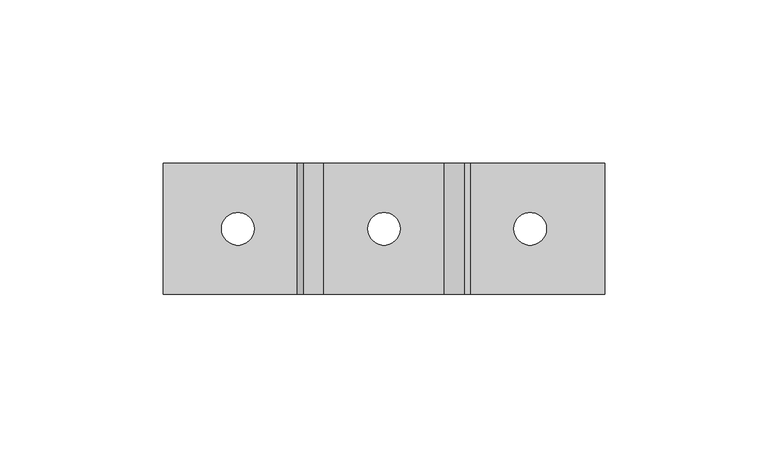
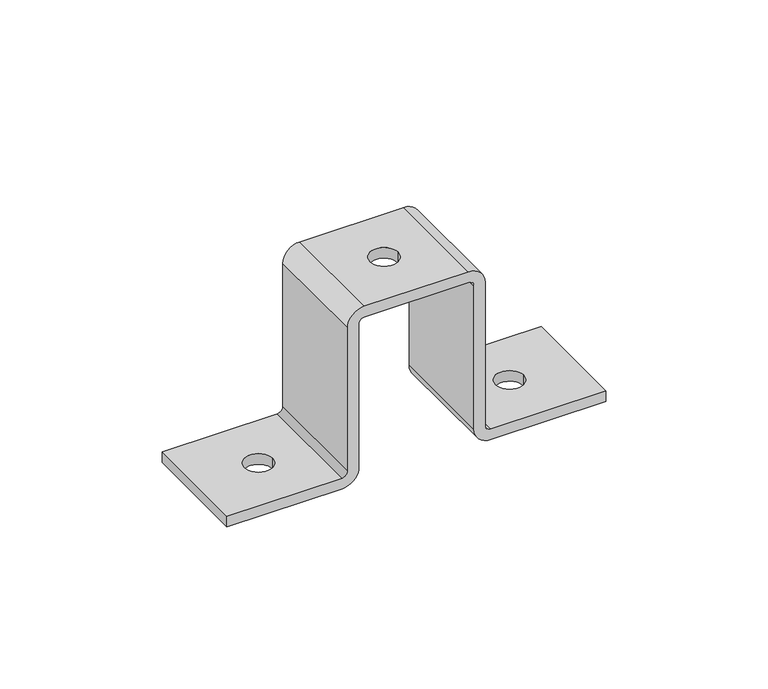
"""IFC4 building model written with IfcOpenShell, lengths in millimetres: proxy geometry, ▶ TN_Скоба соединительная (сборка тип 1) : ▶ TN_Скоба соединительная (сборка тип 1)."""

from ifc_helpers import new_model, si_unit, frame, origin, place, context, project, spatial, polyline, circle_curve, source, transform, mapped, element, save
from ifc_brep_helpers import plane_surface, cylinder_surface, revolved_surface, advanced_brep


def generic_models_d1ea9576(model_context):
    return source(origin(), model_context, "Body", "AdvancedBrep", [
        advanced_brep(
        [(-26.5, -20.0, 0.0), (-20.5, -20.0, 6.0), (-20.5, -20.0, 60.0), (-18.5, -20.0, 62.0), (18.5, -20.0, 62.0), (20.5, -20.0, 60.0), (20.5, -20.0, 6.0), (26.5, -20.0, 0.0), (67.5, -20.0, 0.0), (67.5, -20.0, 4.0), (26.5, -20.0, 4.0), (24.5, -20.0, 6.0), (24.5, -20.0, 60.0), (18.5, -20.0, 66.0), (-18.5, -20.0, 66.0), (-24.5, -20.0, 60.0), (-24.5, -20.0, 6.0), (-26.5, -20.0, 4.0), (-67.5, -20.0, 4.0), (-67.5, -20.0, 0.0), (-26.5, 20.0, 0.0), (-67.5, 20.0, 0.0), (-67.5, 20.0, 4.0), (-26.5, 20.0, 4.0), (-24.5, 20.0, 6.0), (-24.5, 20.0, 60.0), (-18.5, 20.0, 66.0), (18.5, 20.0, 66.0), (24.5, 20.0, 60.0), (24.5, 20.0, 6.0), (26.5, 20.0, 4.0), (67.5, 20.0, 4.0), (67.5, 20.0, 0.0), (26.5, 20.0, 0.0), (20.5, 20.0, 6.0), (20.5, 20.0, 60.0), (18.5, 20.0, 62.0), (-18.5, 20.0, 62.0), (-20.5, 20.0, 60.0), (-20.5, 20.0, 6.0), (-5.0, 0.0, 62.0), (5.0, 0.0, 62.0), (39.7162685, 0.0, 0.0), (49.7162685, 0.0, 0.0), (49.7162685, 0.0, 4.0), (39.7162685, 0.0, 4.0), (5.0, 0.0, 66.0), (-5.0, 0.0, 66.0), (-39.7162685, 0.0, 4.0), (-49.7162685, 0.0, 4.0), (-49.7162685, 0.0, 0.0), (-39.7162685, 0.0, 0.0)],
        [
            (0, 1, circle_curve(frame((-26.5, -20.0, 6.0), z_axis=(0.0, -1.0, 0.0), x_axis=(0.0, 0.0, -1.0)), 6.0)),
            (1, 2),
            (2, 3, circle_curve(frame((-18.5, -20.0, 60.0), z_axis=(0.0, 1.0, 0.0), x_axis=(0.0, 0.0, -1.0)), 2.0)),
            (3, 4),
            (4, 5, circle_curve(frame((18.5, -20.0, 60.0), z_axis=(0.0, 1.0, 0.0), x_axis=(0.0, 0.0, -1.0)), 2.0)),
            (5, 6),
            (6, 7, circle_curve(frame((26.5, -20.0, 6.0), z_axis=(0.0, -1.0, 0.0), x_axis=(0.0, 0.0, -1.0)), 6.0)),
            (7, 8),
            (8, 9),
            (9, 10),
            (10, 11, circle_curve(frame((26.5, -20.0, 6.0), z_axis=(0.0, 1.0, 0.0), x_axis=(0.0, 0.0, -1.0)), 2.0)),
            (11, 12),
            (12, 13, circle_curve(frame((18.5, -20.0, 60.0), z_axis=(0.0, -1.0, 0.0), x_axis=(0.0, 0.0, -1.0)), 6.0)),
            (13, 14),
            (14, 15, circle_curve(frame((-18.5, -20.0, 60.0), z_axis=(0.0, -1.0, 0.0), x_axis=(0.0, 0.0, -1.0)), 6.0)),
            (15, 16),
            (16, 17, circle_curve(frame((-26.5, -20.0, 6.0), z_axis=(0.0, 1.0, 0.0), x_axis=(0.0, 0.0, -1.0)), 2.0)),
            (17, 18),
            (18, 19),
            (19, 0),
            (20, 21),
            (21, 22),
            (22, 23),
            (23, 24, circle_curve(frame((-26.5, 20.0, 6.0), z_axis=(0.0, -1.0, 0.0), x_axis=(0.0, 0.0, -1.0)), 2.0)),
            (24, 25),
            (25, 26, circle_curve(frame((-18.5, 20.0, 60.0), z_axis=(0.0, 1.0, 0.0), x_axis=(0.0, 0.0, -1.0)), 6.0)),
            (26, 27),
            (27, 28, circle_curve(frame((18.5, 20.0, 60.0), z_axis=(0.0, 1.0, 0.0), x_axis=(0.0, 0.0, -1.0)), 6.0)),
            (28, 29),
            (29, 30, circle_curve(frame((26.5, 20.0, 6.0), z_axis=(0.0, -1.0, 0.0), x_axis=(0.0, 0.0, -1.0)), 2.0)),
            (30, 31),
            (31, 32),
            (32, 33),
            (33, 34, circle_curve(frame((26.5, 20.0, 6.0), z_axis=(0.0, 1.0, 0.0), x_axis=(0.0, 0.0, -1.0)), 6.0)),
            (34, 35),
            (35, 36, circle_curve(frame((18.5, 20.0, 60.0), z_axis=(0.0, -1.0, 0.0), x_axis=(0.0, 0.0, -1.0)), 2.0)),
            (36, 37),
            (37, 38, circle_curve(frame((-18.5, 20.0, 60.0), z_axis=(0.0, -1.0, 0.0), x_axis=(0.0, 0.0, -1.0)), 2.0)),
            (38, 39),
            (39, 20, circle_curve(frame((-26.5, 20.0, 6.0), z_axis=(0.0, 1.0, 0.0), x_axis=(0.0, 0.0, -1.0)), 6.0)),
            (0, 20),
            (39, 1),
            (38, 2),
            (37, 3),
            (36, 4),
            (40, 41, circle_curve(frame((0.0, 0.0, 62.0), z_axis=(0.0, 0.0, 1.0), x_axis=(1.0, 0.0, 0.0)), 5.0)),
            (41, 40, circle_curve(frame((0.0, 0.0, 62.0), z_axis=(0.0, 0.0, 1.0), x_axis=(1.0, 0.0, 0.0)), 5.0)),
            (35, 5),
            (34, 6),
            (33, 7),
            (32, 8),
            (42, 43, circle_curve(frame((44.7162685, 0.0, 0.0), z_axis=(0.0, 0.0, 1.0), x_axis=(1.0, 0.0, 0.0)), 5.0)),
            (43, 42, circle_curve(frame((44.7162685, 0.0, 0.0), z_axis=(0.0, 0.0, 1.0), x_axis=(1.0, 0.0, 0.0)), 5.0)),
            (31, 9),
            (30, 10),
            (44, 45, circle_curve(frame((44.7162685, 0.0, 4.0), z_axis=(0.0, 0.0, -1.0), x_axis=(1.0, 0.0, 0.0)), 5.0)),
            (45, 44, circle_curve(frame((44.7162685, 0.0, 4.0), z_axis=(0.0, 0.0, -1.0), x_axis=(1.0, 0.0, 0.0)), 5.0)),
            (29, 11),
            (28, 12),
            (27, 13),
            (26, 14),
            (46, 47, circle_curve(frame((0.0, 0.0, 66.0), z_axis=(0.0, 0.0, -1.0), x_axis=(1.0, 0.0, 0.0)), 5.0)),
            (47, 46, circle_curve(frame((0.0, 0.0, 66.0), z_axis=(0.0, 0.0, -1.0), x_axis=(1.0, 0.0, 0.0)), 5.0)),
            (25, 15),
            (24, 16),
            (23, 17),
            (22, 18),
            (48, 49, circle_curve(frame((-44.7162685, 0.0, 4.0), z_axis=(0.0, 0.0, -1.0), x_axis=(1.0, 0.0, 0.0)), 5.0)),
            (49, 48, circle_curve(frame((-44.7162685, 0.0, 4.0), z_axis=(0.0, 0.0, -1.0), x_axis=(1.0, 0.0, 0.0)), 5.0)),
            (21, 19),
            (50, 51, circle_curve(frame((-44.7162685, 0.0, 0.0), z_axis=(0.0, 0.0, 1.0), x_axis=(1.0, 0.0, 0.0)), 5.0)),
            (51, 50, circle_curve(frame((-44.7162685, 0.0, 0.0), z_axis=(0.0, 0.0, 1.0), x_axis=(1.0, 0.0, 0.0)), 5.0)),
            (48, 51),
            (50, 49),
            (44, 43),
            (42, 45),
            (40, 47),
            (46, 41),
        ],
        [
            plane_surface(frame((0.0, -20.0, 0.0), z_axis=(0.0, -1.0, 0.0), x_axis=(0.0, 0.0, 1.0))),
            plane_surface(frame((0.0, 20.0, 0.0), z_axis=(0.0, 1.0, 0.0), x_axis=(0.0, 0.0, 1.0))),
            cylinder_surface(frame((-26.5, -20.0, 6.0), z_axis=(0.0, -1.0, 0.0), x_axis=(0.0, 0.0, -1.0)), 6.0),
            plane_surface(frame((-20.5, -20.0, 6.0), z_axis=(1.0, 0.0, 0.0), x_axis=(0.0, 1.0, 0.0))),
            revolved_surface(polyline([(-18.5, 20.0, 58.0), (-18.5, -20.0, 58.0)]), (-18.5, -20.0, 60.0), (0.0, 1.0, 0.0)),
            plane_surface(frame((-18.5, -20.0, 62.0), z_axis=(0.0, 0.0, -1.0), x_axis=(0.0, 1.0, 0.0))),
            revolved_surface(polyline([(18.5, 20.0, 58.0), (18.5, -20.0, 58.0)]), (18.5, -20.0, 60.0), (0.0, 1.0, 0.0)),
            plane_surface(frame((20.5, -20.0, 60.0), z_axis=(-1.0, 0.0, 0.0), x_axis=(0.0, 1.0, 0.0))),
            cylinder_surface(frame((26.5, -20.0, 6.0), z_axis=(0.0, -1.0, 0.0), x_axis=(0.0, 0.0, -1.0)), 6.0),
            plane_surface(frame((26.5, -20.0, 0.0), z_axis=(0.0, 0.0, -1.0), x_axis=(0.0, 1.0, 0.0))),
            plane_surface(frame((67.5, -20.0, 0.0), z_axis=(1.0, 0.0, 0.0), x_axis=(0.0, 1.0, 0.0))),
            plane_surface(frame((67.5, -20.0, 4.0), z_axis=(0.0, 0.0, 1.0), x_axis=(0.0, 1.0, 0.0))),
            revolved_surface(polyline([(26.5, 20.0, 4.0), (26.5, -20.0, 4.0)]), (26.5, -20.0, 6.0), (0.0, 1.0, 0.0)),
            plane_surface(frame((24.5, -20.0, 6.0), z_axis=(1.0, 0.0, 0.0), x_axis=(0.0, 1.0, 0.0))),
            cylinder_surface(frame((18.5, -20.0, 60.0), z_axis=(0.0, -1.0, 0.0), x_axis=(0.0, 0.0, -1.0)), 6.0),
            plane_surface(frame((18.5, -20.0, 66.0), z_axis=(0.0, 0.0, 1.0), x_axis=(0.0, 1.0, 0.0))),
            cylinder_surface(frame((-18.5, -20.0, 60.0), z_axis=(0.0, -1.0, 0.0), x_axis=(0.0, 0.0, -1.0)), 6.0),
            plane_surface(frame((-24.5, -20.0, 60.0), z_axis=(-1.0, 0.0, 0.0), x_axis=(0.0, 1.0, 0.0))),
            revolved_surface(polyline([(-26.5, 20.0, 4.0), (-26.5, -20.0, 4.0)]), (-26.5, -20.0, 6.0), (0.0, 1.0, 0.0)),
            plane_surface(frame((-26.5, -20.0, 4.0), z_axis=(0.0, 0.0, 1.0), x_axis=(0.0, 1.0, 0.0))),
            plane_surface(frame((-67.5, -20.0, 4.0), z_axis=(-1.0, 0.0, 0.0), x_axis=(0.0, 1.0, 0.0))),
            plane_surface(frame((-67.5, -20.0, 0.0), z_axis=(0.0, 0.0, -1.0), x_axis=(0.0, 1.0, 0.0))),
            revolved_surface(polyline([(-39.7162685, 0.0, 4.0), (-39.7162685, 0.0, 0.0)]), (-44.7162685, 0.0, 0.0), (0.0, 0.0, 1.0)),
            revolved_surface(polyline([(49.7162685, 0.0, 4.0), (49.7162685, 0.0, 0.0)]), (44.7162685, 0.0, 0.0), (0.0, 0.0, 1.0)),
            revolved_surface(polyline([(5.0, 0.0, 66.0), (5.0, 0.0, 62.0)]), (0.0, 0.0, 35.2036226), (0.0, 0.0, 1.0)),
        ],
        [
            (0, [[1, 2, 3, 4, 5, 6, 7, 8, 9, 10, 11, 12, 13, 14, 15, 16, 17, 18, 19, 20]]),
            (1, [[21, 22, 23, 24, 25, 26, 27, 28, 29, 30, 31, 32, 33, 34, 35, 36, 37, 38, 39, 40]]),
            (2, [[-1, 41, -40, 42]]),
            (3, [[-2, -42, -39, 43]]),
            (4, [[-3, -43, -38, 44]]),
            (5, [[-4, -44, -37, 45], [46, 47]]),
            (6, [[-5, -45, -36, 48]]),
            (7, [[-6, -48, -35, 49]]),
            (8, [[-7, -49, -34, 50]]),
            (9, [[-8, -50, -33, 51], [52, 53]]),
            (10, [[-9, -51, -32, 54]]),
            (11, [[-10, -54, -31, 55], [56, 57]]),
            (12, [[-11, -55, -30, 58]]),
            (13, [[-12, -58, -29, 59]]),
            (14, [[-13, -59, -28, 60]]),
            (15, [[-14, -60, -27, 61], [62, 63]]),
            (16, [[-15, -61, -26, 64]]),
            (17, [[-16, -64, -25, 65]]),
            (18, [[-17, -65, -24, 66]]),
            (19, [[-18, -66, -23, 67], [68, 69]]),
            (20, [[-19, -67, -22, 70]]),
            (21, [[-20, -70, -21, -41], [71, 72]]),
            (22, [[73, -71, 74, -68]]),
            (22, [[-73, -69, -74, -72]]),
            (23, [[75, -52, 76, -56]]),
            (23, [[-75, -57, -76, -53]]),
            (24, [[77, -62, 78, -46]]),
            (24, [[-77, -47, -78, -63]]),
        ],
    ),
    ])


if __name__ == "__main__":
    model = new_model("IFC4")
    model_context = context("Model", 3, world=origin())
    ifc_project = project(units=[si_unit("LENGTHUNIT", "METRE", prefix="MILLI")], contexts=[model_context])
    site = spatial("IfcSite", under=ifc_project)
    building = spatial("IfcBuilding", under=site)
    placement = place(None, origin())
    generic_models_shape = generic_models_d1ea9576(model_context)
    element("IfcBuildingElementProxy", 1, Name="▶ TN_Скоба соединительная (сборка тип 1) : ▶ TN_Скоба соединительная (сборка тип 1)", ObjectType="▶ TN_Скоба соединительная (сборка тип 1) : ▶ TN_Скоба соединительная (сборка тип 1)", at=placement, inside=building, context=model_context, shape_type="MappedRepresentation", body=[
        mapped(generic_models_shape, transform((0.0, 0.0, 0.0), x_axis=(1.0, 0.0, 0.0), y_axis=(0.0, 1.0, 0.0), z_axis=(0.0, 0.0, 1.0))),
    ])
    save(model, "model.ifc")

# Revit data of these elements
# Type "▶ TN_Скоба соединительная (сборка тип 1) : ▶ TN_Скоба соединительная (сборка тип 1)"
#   Description = "Cоединительный элемент для монтажа рам, стеллажей, каркасов для легких и средних систем. Обеспечивает устойчивое поперечное (крестовое) соединение профилей. Наиболее эффективно использования скобы, как соединителя для создания пространственных силовых, опорных каркасов и решеток. Возможность реализации крепления профиля к бетонному основанию."
#   Manufacturer = "ТехноНИКОЛЬ"
#   Model = "Комплектующие к опорам"
#   URL = "https://nav.tn.ru/knowledge-base/polimernye-membrany/opory-pod-oborudovanie-na-ploskoy-krovle/?sphrase_id=266812"
#   ADSK_Обозначение = "ТехноНИКОЛЬ"
#   ADSK_Наименование краткое [instance default] = "С41х124 4F3"
#   ADSK_Наименование [instance default] = "Скоба соединительная 41х124 4F3"
#   ADSK_Масса_Текст = ""
#   ADSK_Марка [instance default] = "С41х124 4F3"
#   ADSK_Код изделия [instance default] = "690885"
#   ADSK_Завод-изготовитель = "ТехноНИКОЛЬ"
#   ADSK_Единица измерения = "шт."
#   ADSK_Группирование = "Комплектующие к опорам"
#   ADSK_URL страницы изделия = "https://nav.tn.ru/knowledge-base/polimernye-membrany/opory-pod-oborudovanie-na-ploskoy-krovle/?sphrase_id=266812"
#   ADSK_URL документации изделия = ""
#   Высота крепежа [instance default] = 84 mm
#   ADSK_Количество = 1
#   Скоба соединительная 41х62 4F3 [instance default] = no
#   Скоба соединительная 41х41 4F5 [instance default] = no
#   Скоба соединительная 41х124 4F3 [instance default] = yes
#   ADSK_Материал = TN_СтальГальванизированная_Серый
#   Default Elevation = 0
# Element 1 (IfcBuildingElementProxy, "▶ TN_Скоба соединительная (сборка тип 1) : ▶ TN_Скоба соединительная (сборка тип 1)")
#   ADSK_Наименование краткое = "С41х62 4F3"
#   ADSK_Наименование = "Скоба соединительная 41х62 4F3"
#   ADSK_Марка = "С41х62 4F3"
#   ADSK_Код изделия = "660819"
#   Высота крепежа = 22 mm
#   Скоба соединительная 41х62 4F3 = yes
#   Скоба соединительная 41х124 4F3 = no
#   Materials on its faces: "TN_СтальГальванизированная_Серый"
# Materials
#   "TN_СтальГальванизированная_Серый": class "Типовые", colour RGB 206 210 213, transparency 0, Cost = 0
